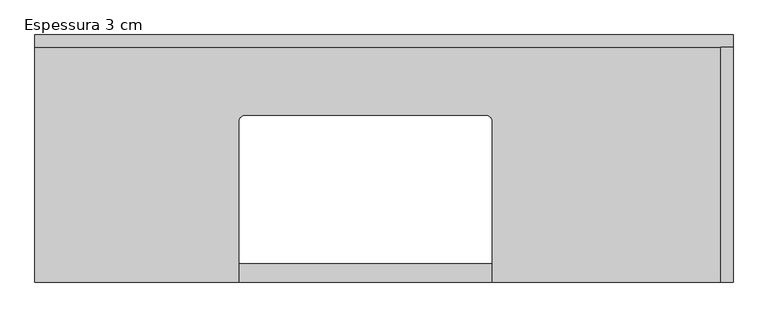
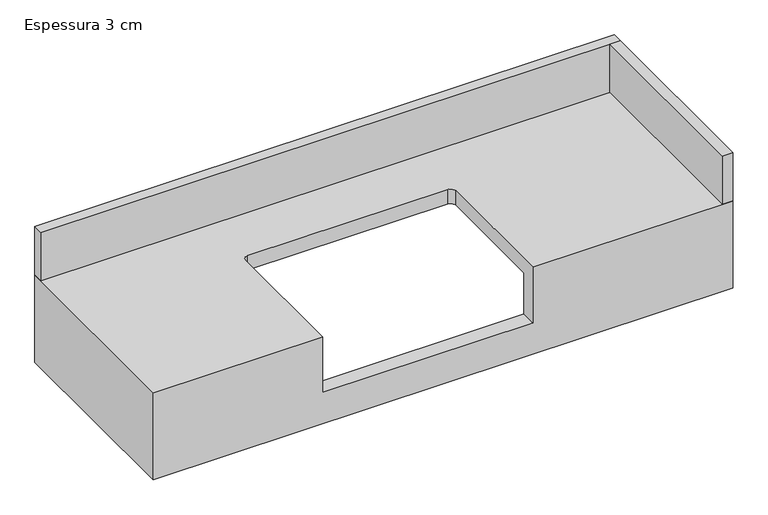
"""IFC4 building model written with IfcOpenShell, lengths in millimetres: furniture geometry, CC_BANCADA BANHEIRO COM CUBA_CANTO RETO : Espessura 3 cm."""

from ifc_helpers import new_model, si_unit, frame, origin, place, context, project, spatial, polyline, circle_curve, outline, extrude, source, transform, mapped, element, save
from ifc_brep_helpers import plane_surface, revolved_surface, advanced_brep


def espessura_3_cm_f12d49ab(model_context):
    return source(origin(), model_context, "Body", "SolidModel", [
        advanced_brep(
        [(750.0, 300.0, 860.0), (-380.0, 300.0, 860.0), (-380.0, -100.0, 860.0), (-50.0, -100.0, 860.0), (-50.0, 160.0, 860.0), (-40.0, 170.0, 860.0), (350.0, 170.0, 860.0), (360.0, 160.0, 860.0), (360.0, -100.0, 860.0), (750.0, -100.0, 860.0), (750.0, 300.0, 680.0), (720.0, 300.0, 680.0), (720.0, 300.0, 830.0), (-350.0, 300.0, 830.0), (-350.0, 300.0, 680.0), (-380.0, 300.0, 680.0), (-380.0, -100.0, 680.0), (750.0, -100.0, 680.0), (360.0, -100.0, 745.0), (-50.0, -100.0, 745.0), (720.0, -70.0, 830.0), (360.0, -70.0, 830.0), (360.0, 160.0, 830.0), (350.0, 170.0, 830.0), (-40.0, 170.0, 830.0), (-50.0, 160.0, 830.0), (-50.0, -70.0, 830.0), (-350.0, -70.0, 830.0), (-350.0, -70.0, 680.0), (-50.0, -70.0, 745.0), (360.0, -70.0, 745.0), (720.0, -70.0, 680.0)],
        [
            (0, 1),
            (1, 2),
            (2, 3),
            (3, 4),
            (4, 5, circle_curve(frame((-40.0, 160.0, 860.0), z_axis=(0.0, 0.0, -1.0), x_axis=(0.0, 1.0, 0.0)), 10.0)),
            (5, 6),
            (6, 7, circle_curve(frame((350.0, 160.0, 860.0), z_axis=(0.0, 0.0, -1.0), x_axis=(0.0, 1.0, 0.0)), 10.0)),
            (7, 8),
            (8, 9),
            (9, 0),
            (0, 10),
            (10, 11),
            (11, 12),
            (12, 13),
            (13, 14),
            (14, 15),
            (15, 1),
            (15, 16),
            (16, 2),
            (16, 17),
            (17, 9),
            (8, 18),
            (18, 19),
            (19, 3),
            (17, 10),
            (12, 20),
            (20, 21),
            (21, 22),
            (22, 23, circle_curve(frame((350.0, 160.0, 830.0), z_axis=(0.0, 0.0, 1.0), x_axis=(0.0, 1.0, 0.0)), 10.0)),
            (23, 24),
            (24, 25, circle_curve(frame((-40.0, 160.0, 830.0), z_axis=(0.0, 0.0, 1.0), x_axis=(0.0, 1.0, 0.0)), 10.0)),
            (25, 26),
            (26, 27),
            (27, 13),
            (27, 28),
            (28, 14),
            (26, 29),
            (29, 30),
            (30, 21),
            (20, 31),
            (31, 28),
            (11, 31),
            (5, 24),
            (23, 6),
            (18, 30),
            (29, 19),
            (4, 25),
            (7, 22),
        ],
        [
            plane_surface(frame((-380.0, 300.0, 860.0), z_axis=(0.0, 0.0, 1.0), x_axis=(-1.0, 0.0, 0.0))),
            plane_surface(frame((750.0, 300.0, 860.0), z_axis=(0.0, 1.0, 0.0), x_axis=(0.0, 0.0, -1.0))),
            plane_surface(frame((-380.0, 300.0, 860.0), z_axis=(-1.0, 0.0, 0.0), x_axis=(0.0, 0.0, -1.0))),
            plane_surface(frame((-380.0, -100.0, 860.0), z_axis=(0.0, -1.0, 0.0), x_axis=(0.0, 0.0, -1.0))),
            plane_surface(frame((750.0, -100.0, 860.0), z_axis=(1.0, 0.0, 0.0), x_axis=(0.0, 0.0, -1.0))),
            plane_surface(frame((-350.0, 300.0, 830.0), z_axis=(0.0, 0.0, -1.0), x_axis=(-1.0, 0.0, 0.0))),
            plane_surface(frame((-350.0, 300.0, 830.0), z_axis=(1.0, 0.0, 0.0), x_axis=(0.0, 0.0, -1.0))),
            plane_surface(frame((-350.0, -70.0, 830.0), z_axis=(0.0, 1.0, 0.0), x_axis=(0.0, 0.0, -1.0))),
            plane_surface(frame((720.0, -70.0, 830.0), z_axis=(-1.0, 0.0, 0.0), x_axis=(0.0, 0.0, -1.0))),
            plane_surface(frame((750.0, -100.0, 680.0), z_axis=(0.0, 0.0, -1.0), x_axis=(0.0, 1.0, 0.0))),
            plane_surface(frame((-40.0, 170.0, 745.0), z_axis=(0.0, -1.0, 0.0), x_axis=(0.0, 0.0, 1.0))),
            plane_surface(frame((350.0, 170.0, 745.0), z_axis=(0.0, 0.0, 1.0), x_axis=(1.0, 0.0, 0.0))),
            revolved_surface(polyline([(-40.0, 170.0, 830.0), (-40.0, 170.0, 860.0)]), (-40.0, 160.0, 900.0), (0.0, 0.0, -1.0)),
            plane_surface(frame((-50.0, -230.0, 745.0), z_axis=(1.0, 0.0, 0.0), x_axis=(0.0, 0.0, 1.0))),
            plane_surface(frame((360.0, 160.0, 745.0), z_axis=(-1.0, 0.0, 0.0), x_axis=(0.0, 0.0, 1.0))),
            revolved_surface(polyline([(350.0, 170.0, 830.0), (350.0, 170.0, 860.0)]), (350.0, 160.0, 900.0), (0.0, 0.0, -1.0)),
        ],
        [
            (0, [[1, 2, 3, 4, 5, 6, 7, 8, 9, 10]]),
            (1, [[-1, 11, 12, 13, 14, 15, 16, 17]]),
            (2, [[-2, -17, 18, 19]]),
            (3, [[-3, -19, 20, 21, -9, 22, 23, 24]]),
            (4, [[-10, -21, 25, -11]]),
            (5, [[26, 27, 28, 29, 30, 31, 32, 33, 34, -14]]),
            (6, [[-34, 35, 36, -15]]),
            (7, [[-33, 37, 38, 39, -27, 40, 41, -35]]),
            (8, [[-26, -13, 42, -40]]),
            (9, [[-12, -25, -20, -18, -16, -36, -41, -42]]),
            (10, [[-6, 43, -30, 44]]),
            (11, [[-23, 45, -38, 46]]),
            (12, [[-5, 47, -31, -43]]),
            (13, [[-4, -24, -46, -37, -32, -47]]),
            (14, [[-8, 48, -28, -39, -45, -22]]),
            (15, [[-7, -44, -29, -48]]),
        ],
    ),
        extrude(outline(polyline([(730.0, 280.0), (750.0, 280.0), (750.0, -100.0), (730.0, -100.0), (730.0, 280.0)])), frame((0.0, 0.0, 860.0), z_axis=(0.0, 0.0, 1.0), x_axis=(1.0, 0.0, 0.0)), (0.0, 0.0, 1.0), 100.0),
        extrude(outline(polyline([(750.0, 300.0), (750.0, 280.0), (-380.0, 280.0), (-380.0, 300.0), (750.0, 300.0)])), frame((0.0, 0.0, 860.0), z_axis=(0.0, 0.0, 1.0), x_axis=(1.0, 0.0, 0.0)), (0.0, 0.0, 1.0), 100.0),
    ])


if __name__ == "__main__":
    model = new_model("IFC4")
    model_context = context("Model", 3, world=origin())
    ifc_project = project(units=[si_unit("LENGTHUNIT", "METRE", prefix="MILLI")], contexts=[model_context])
    site = spatial("IfcSite", under=ifc_project)
    building = spatial("IfcBuilding", under=site)
    placement = place(None, origin())
    espessura_3_cm_shape = espessura_3_cm_f12d49ab(model_context)
    element("IfcFurniture", 1, ObjectType="CC_BANCADA BANHEIRO COM CUBA_CANTO RETO : Espessura 3 cm", at=placement, inside=building, context=model_context, shape_type="MappedRepresentation", body=[
        mapped(espessura_3_cm_shape, transform((0.0, 0.0, 0.0), x_axis=(1.0, 0.0, 0.0), y_axis=(0.0, 1.0, 0.0), z_axis=(0.0, 0.0, 1.0))),
    ])
    save(model, "model.ifc")

# Revit data of these elements
# Type "CC_BANCADA BANHEIRO COM CUBA_CANTO RETO : Espessura 3 cm"
#   Uso HS [instance default] = ""
#   h TESTEIRA AUX [instance default] = 0.15 m
#   Altura testeira [instance default] = 0.15 m
#   Altura rodapia [instance default] = 0.10 m
#   Espessura rodapia [instance default] = 0.02 m
#   Prof/2 [instance default] = 0.20 m
#   Offset cuba esquerda [instance default] = 0.40 m
#   Depth [instance default] = 1.20 m
#   Width [instance default] = 0.40 m
#   Espessura bancada = 0.03 m
#   Comprimento [instance default] = 1.20 m
#   Height [instance default] = 0.86 m
#   Testeira [instance default] = yes
#   Rodapia fundo [instance default] = no
#   Rodapia esquerda [instance default] = no
#   Rodapia direita [instance default] = no
#   Material porta-toalha [instance default] = .CROMADO
#   Material hidráulico [instance default] = .CROMADO
#   Material cuba [instance default] = .PORCELANA BRANCA
#   Material bancada [instance default] = .GRANITO_BRANCO_ITAUNAS
#   Assembly Code = ""
# Element 1 (IfcFurniture, "CC_BANCADA BANHEIRO COM CUBA_CANTO RETO : Espessura 3 cm")
#   Uso HS = "BANHO SUÍTE 1"
#   Offset cuba esquerda = 0.33 m
#   Depth = 1.13 m
#   Comprimento = 1.13 m
#   Rodapia fundo = yes
#   Rodapia direita = yes
#   Materials on its faces: ".GRANITO_BRANCO_ITAUNAS"
# Materials
#   ".CROMADO": class "CC_METAIS", colour RGB 211 223 226, transparency 0, Cost = 0
#   ".PORCELANA BRANCA": class "CC_PORCELANA", colour RGB 230 230 230, transparency 0, Cost = 0
#   ".GRANITO_BRANCO_ITAUNAS": class ".CC_PEDRA REVEST.", colour RGB 202 195 174, transparency 0, Description = "Revestimento em granito", Cost = 0
